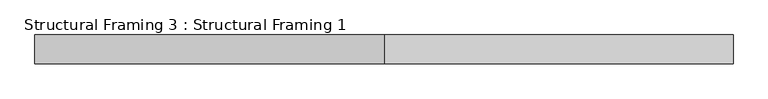
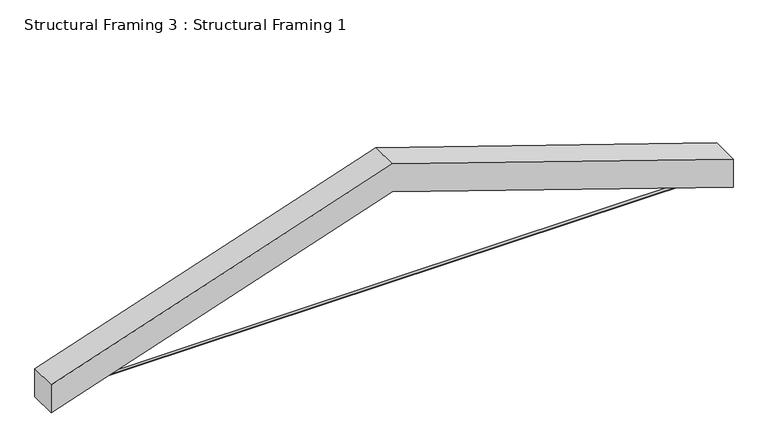
"""IFC4 building model written with IfcOpenShell, lengths in millimetres: beam geometry, Structural Framing 3 : Structural Framing 1."""

from ifc_helpers import new_model, si_unit, point, frame, frame_2d, origin, place, context, project, spatial, polyline, circle_curve, trimmed, segment, composite_curve, outline, extrude, source, transform, mapped, element, save


def structural_framing_3_structural_framing_1_e19fbcf0(model_context):
    return source(origin(), model_context, "Body", "SweptSolid", [
        extrude(outline(composite_curve([segment(trimmed(circle_curve(frame_2d((172.7115366, 4984.3019529)), 6.35), [point((179.0615366, 4984.3019529))], [point((166.3615366, 4984.3019529))], False, "CARTESIAN"), True, "CONTINUOUS"), segment(trimmed(circle_curve(frame_2d((172.7115366, 4984.3019529)), 6.35), [point((166.3615366, 4984.3019529))], [point((179.0615366, 4984.3019529))], False, "CARTESIAN"), True, "CONTINUOUS")], self_intersect=False)), frame((19888.9870052, 0.0, 0.0), z_axis=(1.0, 0.0, 0.0), x_axis=(0.0, 1.0, 0.0)), (0.0, 0.0, 1.0), 3111.5),
        extrude(outline(polyline([(5652.475838, 21444.7370052), (5084.8528105, 19749.2870052), (4937.5315162, 19749.2870052), (5505.1545437, 21444.7370052), (4937.5315162, 23140.1870052), (5084.8528105, 23140.1870052), (5652.475838, 21444.7370052)])), frame((0.0, 102.8615366, 0.0), z_axis=(0.0, 1.0, 0.0), x_axis=(0.0, 0.0, 1.0)), (0.0, 0.0, 1.0), 139.7),
    ])


if __name__ == "__main__":
    model = new_model("IFC4")
    model_context = context("Model", 3, world=origin())
    ifc_project = project(units=[si_unit("LENGTHUNIT", "METRE", prefix="MILLI")], contexts=[model_context])
    site = spatial("IfcSite", under=ifc_project)
    building = spatial("IfcBuilding", under=site)
    placement = place(None, origin())
    structural_framing_3_structural_framing_1_shape = structural_framing_3_structural_framing_1_e19fbcf0(model_context)
    element("IfcBeam", 1, ObjectType="Structural Framing 3 : Structural Framing 1", at=placement, inside=building, context=model_context, shape_type="MappedRepresentation", body=[
        mapped(structural_framing_3_structural_framing_1_shape, transform((0.0, 0.0, 0.0), x_axis=(1.0, 0.0, 0.0), y_axis=(0.0, 1.0, 0.0), z_axis=(0.0, 0.0, 1.0))),
    ])
    save(model, "model.ifc")

# Revit data of these elements
# Element 1 (IfcBeam, "Structural Framing 3 : Structural Framing 1")
#   Materials on its faces: "GLULAM TRUSS W/ CUSTOM GUSSET PLATES", "COLLAR TIE: 1/2\" GALV. ROD"
# Materials
#   "GLULAM TRUSS W/ CUSTOM GUSSET PLATES": class "Generic", colour RGB 206 153 90, transparency 0, Cost = 0
#   "COLLAR TIE: 1/2\" GALV. ROD": class "Generic", colour RGB 49 49 49, transparency 0, Cost = 0
